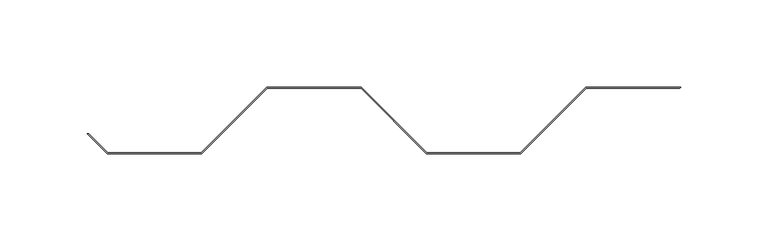
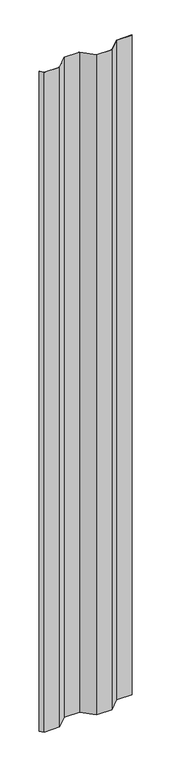
"""IFC4 building model written with IfcOpenShell, lengths in millimetres: proxy geometry, MBCI 7.2-V Panel1 : MBCI 7.2-V Panel-1."""

from ifc_helpers import new_model, si_unit, origin, origin_with_axes, place, context, project, spatial, polyline, outline, extrude, source, transform, mapped, element, save


def generic_models_00b0cba8(model_context):
    return source(origin(), model_context, "Body", "SweptSolid", [
        extrude(outline(polyline([(590069.9303729, -531639.2163841), (590015.8186638, -531639.2163841), (590004.4180296, -531627.81575), (590005.2180038, -531627.7738251), (590016.0652503, -531638.6210716), (590069.6837864, -531638.6210716), (590107.1741864, -531601.1306716), (590161.4548503, -531601.1306716), (590198.9452503, -531638.6210716), (590252.5637864, -531638.6210716), (590290.0541864, -531601.1306716), (590344.3348503, -531601.1306716), (590343.7395378, -531601.7259841), (590290.3007729, -531601.7259841), (590252.8103729, -531639.2163841), (590198.6986638, -531639.2163841), (590161.2082638, -531601.7259841), (590107.4207729, -531601.7259841), (590069.9303729, -531639.2163841)])), origin_with_axes(), (0.0, 0.0, 1.0), 2438.4),
    ])


if __name__ == "__main__":
    model = new_model("IFC4")
    model_context = context("Model", 3, world=origin())
    ifc_project = project(units=[si_unit("LENGTHUNIT", "METRE", prefix="MILLI")], contexts=[model_context])
    site = spatial("IfcSite", under=ifc_project)
    building = spatial("IfcBuilding", under=site)
    placement = place(None, origin())
    generic_models_shape = generic_models_00b0cba8(model_context)
    element("IfcBuildingElementProxy", 1, Name="MBCI 7.2-V Panel1 : MBCI 7.2-V Panel-1", ObjectType="MBCI 7.2-V Panel1 : MBCI 7.2-V Panel-1", at=placement, inside=building, context=model_context, shape_type="MappedRepresentation", body=[
        mapped(generic_models_shape, transform((0.0, 0.0, 0.0), x_axis=(1.0, 0.0, 0.0), y_axis=(0.0, 1.0, 0.0), z_axis=(0.0, 0.0, 1.0))),
    ])
    save(model, "model.ifc")

# Revit data of these elements
# Project information
#   Project Issue Date = "Issue Date"
#   Project Status = "Project Status"
#   Client Name = "Xcel"
#   Project Address = "Enter address here"
#   Project Name = "Sports Complex"
#   Project Number = "Project Number"
# Element 1 (IfcBuildingElementProxy, "MBCI 7.2-V Panel1 : MBCI 7.2-V Panel-1")
#   Materials on its faces: "MTL PANEL"
# Materials
#   "MTL PANEL": class "Generic", colour RGB 239 242 240, transparency 0, Cost = 0
